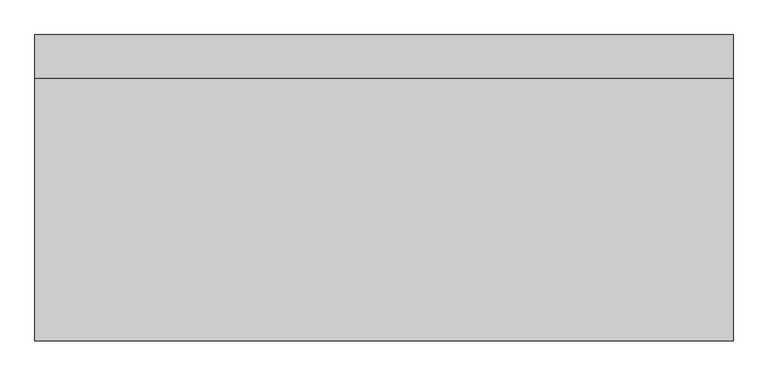
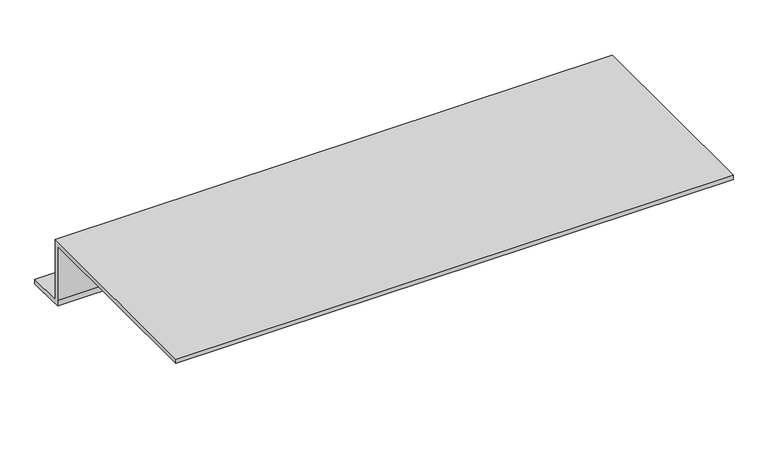
"""IFC4 building model written with IfcOpenShell, lengths in millimetres: proxy geometry, Gypsum013 1411 : Gypsum013 1411."""

from ifc_helpers import new_model, si_unit, frame, origin, place, context, project, spatial, polyline, outline, extrude, source, transform, mapped, element, save


def generic_models_db936d51(model_context):
    return source(origin(), model_context, "Body", "SweptSolid", [
        extrude(outline(polyline([(9592.4838724, 39528.496), (9718.4918386, 39528.496), (9718.4918386, 39511.842875), (9598.7832673, 39511.842875), (9598.7832673, 39513.122875), (9577.6300834, 39513.122875), (9577.6300834, 39534.2760589), (9576.3500834, 39534.2760589), (9576.3500834, 39740.2037188), (8841.3016459, 39740.2037188), (8841.3016459, 39757.096), (9592.4838724, 39757.096), (9592.4838724, 39528.496)])), frame((3694.2883192, 0.0, 0.0), z_axis=(1.0, 0.0, 0.0), x_axis=(0.0, 1.0, 0.0)), (0.0, 0.0, 1.0), 2000.0),
    ])


if __name__ == "__main__":
    model = new_model("IFC4")
    model_context = context("Model", 3, world=origin())
    ifc_project = project(units=[si_unit("LENGTHUNIT", "METRE", prefix="MILLI")], contexts=[model_context])
    site = spatial("IfcSite", under=ifc_project)
    building = spatial("IfcBuilding", under=site)
    placement = place(None, origin())
    generic_models_shape = generic_models_db936d51(model_context)
    element("IfcBuildingElementProxy", 1, Name="Gypsum013 1411 : Gypsum013 1411", ObjectType="Gypsum013 1411 : Gypsum013 1411", at=placement, inside=building, context=model_context, shape_type="MappedRepresentation", body=[
        mapped(generic_models_shape, transform((0.0, 0.0, 0.0), x_axis=(1.0, 0.0, 0.0), y_axis=(0.0, 1.0, 0.0), z_axis=(0.0, 0.0, 1.0))),
    ])
    save(model, "model.ifc")

# Revit data of these elements
# Type "Gypsum013 1411 : Gypsum013 1411"
#   NameOverride = "Gypsum013"
# Element 1 (IfcBuildingElementProxy, "Gypsum013 1411 : Gypsum013 1411")
#   Materials on its faces: "5/8\"  GYPSUM BOARD"
# Materials
#   "5/8\"  GYPSUM BOARD": class "Unassigned", colour RGB 255 255 255, transparency 0, Cost = 0
